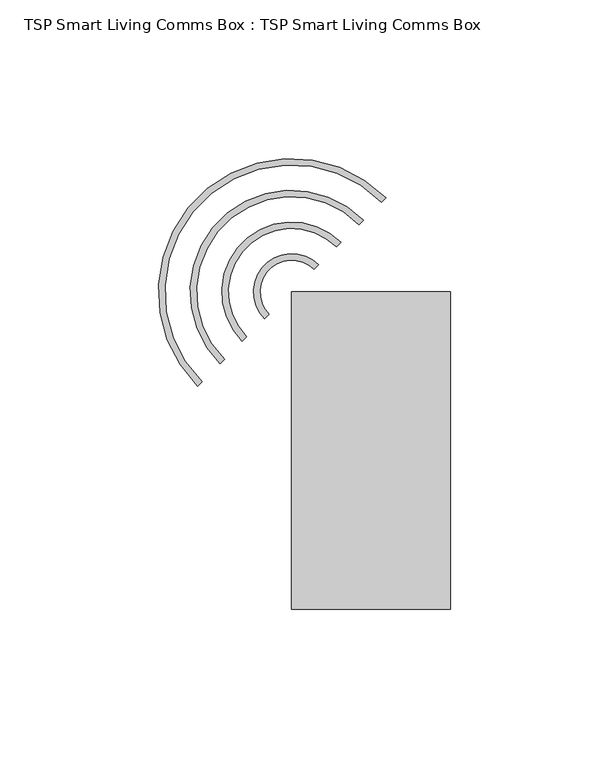
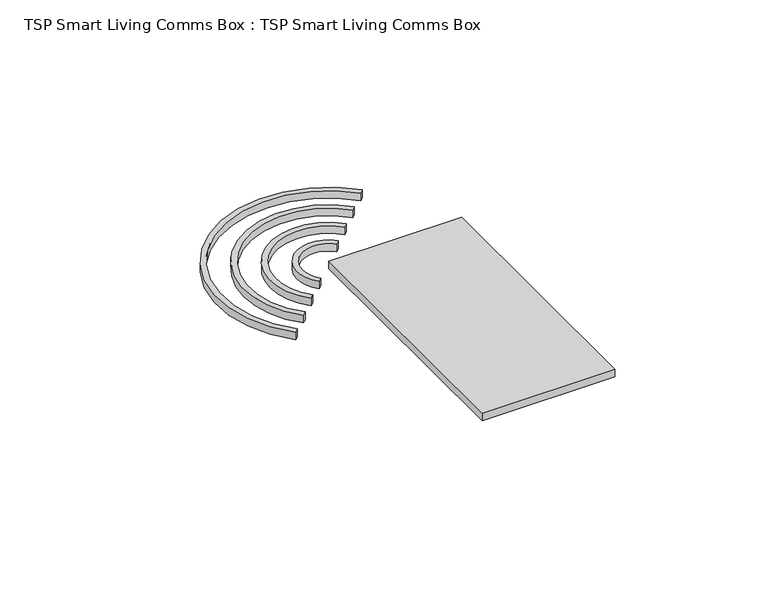
"""IFC4 building model written with IfcOpenShell, lengths in millimetres: proxy geometry, TSP Smart Living Comms Box : TSP Smart Living Comms Box."""

from ifc_helpers import new_model, si_unit, point, frame_2d, origin, origin_with_axes, place, context, project, spatial, polyline, circle_curve, trimmed, segment, composite_curve, outline, extrude, source, transform, mapped, element, save


def tsp_smart_living_comms_box_tsp_smart_living_comms_box_f2f347f1(model_context):
    return source(origin(), model_context, "Body", "SweptSolid", [
        extrude(outline(polyline([(-50.0, 50.0), (0.0, 50.0), (0.0, -50.0), (-50.0, -50.0), (-50.0, 50.0)])), origin_with_axes(), (0.0, 0.0, 1.0), 3.0),
        extrude(outline(composite_curve([segment(polyline([(-78.2842712, 21.7157288), (-79.6984848, 20.3015152)]), True, "CONTINUOUS"), segment(trimmed(circle_curve(frame_2d((-50.0, 50.0)), 42.0), [point((-79.6984848, 20.3015152))], [point((-20.3015152, 79.6984848))], False, "CARTESIAN"), True, "CONTINUOUS"), segment(polyline([(-20.3015152, 79.6984848), (-21.7157288, 78.2842712)]), True, "CONTINUOUS"), segment(trimmed(circle_curve(frame_2d((-50.0, 50.0)), 40.0), [point((-21.7157288, 78.2842712))], [point((-78.2842712, 21.7157288))], True, "CARTESIAN"), True, "CONTINUOUS")], self_intersect=False)), origin_with_axes(), (0.0, 0.0, 1.0), 3.0),
        extrude(outline(composite_curve([segment(polyline([(-27.372583, 72.627417), (-28.7867966, 71.2132034)]), True, "CONTINUOUS"), segment(trimmed(circle_curve(frame_2d((-50.0, 50.0)), 30.0), [point((-28.7867966, 71.2132034))], [point((-71.2132034, 28.7867966))], True, "CARTESIAN"), True, "CONTINUOUS"), segment(polyline([(-71.2132034, 28.7867966), (-72.627417, 27.372583)]), True, "CONTINUOUS"), segment(trimmed(circle_curve(frame_2d((-50.0, 50.0)), 32.0), [point((-72.627417, 27.372583))], [point((-27.372583, 72.627417))], False, "CARTESIAN"), True, "CONTINUOUS")], self_intersect=False)), origin_with_axes(), (0.0, 0.0, 1.0), 3.0),
        extrude(outline(composite_curve([segment(polyline([(-34.4436508, 65.5563492), (-35.8578644, 64.1421356)]), True, "CONTINUOUS"), segment(trimmed(circle_curve(frame_2d((-50.0, 50.0)), 20.0), [point((-35.8578644, 64.1421356))], [point((-64.1421356, 35.8578644))], True, "CARTESIAN"), True, "CONTINUOUS"), segment(polyline([(-64.1421356, 35.8578644), (-65.5563492, 34.4436508)]), True, "CONTINUOUS"), segment(trimmed(circle_curve(frame_2d((-50.0, 50.0)), 22.0), [point((-65.5563492, 34.4436508))], [point((-34.4436508, 65.5563492))], False, "CARTESIAN"), True, "CONTINUOUS")], self_intersect=False)), origin_with_axes(), (0.0, 0.0, 1.0), 3.0),
        extrude(outline(composite_curve([segment(polyline([(-41.5147186, 58.4852814), (-42.9289322, 57.0710678)]), True, "CONTINUOUS"), segment(trimmed(circle_curve(frame_2d((-50.0, 50.0)), 10.0), [point((-42.9289322, 57.0710678))], [point((-57.0710678, 42.9289322))], True, "CARTESIAN"), True, "CONTINUOUS"), segment(polyline([(-57.0710678, 42.9289322), (-58.4852814, 41.5147186)]), True, "CONTINUOUS"), segment(trimmed(circle_curve(frame_2d((-50.0, 50.0)), 12.0), [point((-58.4852814, 41.5147186))], [point((-41.5147186, 58.4852814))], False, "CARTESIAN"), True, "CONTINUOUS")], self_intersect=False)), origin_with_axes(), (0.0, 0.0, 1.0), 3.0),
    ])


if __name__ == "__main__":
    model = new_model("IFC4")
    model_context = context("Model", 3, world=origin())
    ifc_project = project(units=[si_unit("LENGTHUNIT", "METRE", prefix="MILLI")], contexts=[model_context])
    site = spatial("IfcSite", under=ifc_project)
    building = spatial("IfcBuilding", under=site)
    placement = place(None, origin())
    tsp_smart_living_comms_box_tsp_smart_living_comms_box_shape = tsp_smart_living_comms_box_tsp_smart_living_comms_box_f2f347f1(model_context)
    element("IfcBuildingElementProxy", 1, Name="TSP Smart Living Comms Box : TSP Smart Living Comms Box", ObjectType="TSP Smart Living Comms Box : TSP Smart Living Comms Box", at=placement, inside=building, context=model_context, shape_type="MappedRepresentation", body=[
        mapped(tsp_smart_living_comms_box_tsp_smart_living_comms_box_shape, transform((0.0, 0.0, 0.0), x_axis=(1.0, 0.0, 0.0), y_axis=(0.0, 1.0, 0.0), z_axis=(0.0, 0.0, 1.0))),
    ])
    save(model, "model.ifc")

# Revit data of these elements
# Type "TSP Smart Living Comms Box : TSP Smart Living Comms Box"
#   Model = "TSP_ELECSMRTCOMBX"
#   Default Elevation = 0
# Element 1 (IfcBuildingElementProxy, "TSP Smart Living Comms Box : TSP Smart Living Comms Box")
#   Materials on its faces: "Aluminum, Anodized Red"
# Materials
#   "Aluminum, Anodized Red": class "Metal", colour RGB 120 120 120, transparency 0, Description = "Anodized aluminum, red", Cost = 0
